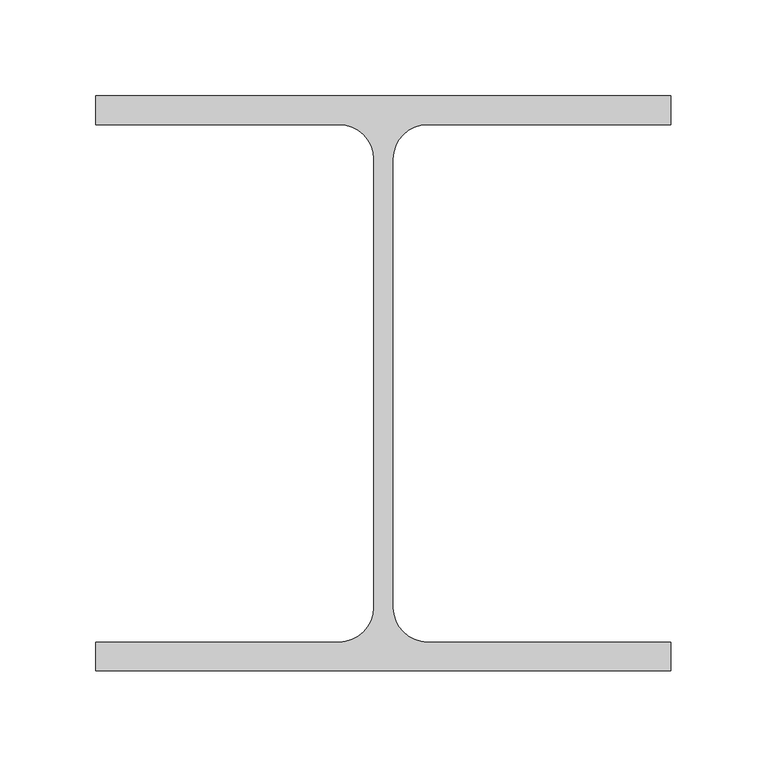
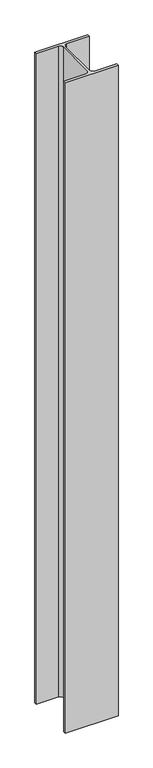
"""IFC4 building model written with IfcOpenShell, lengths in millimetres: column geometry, 0912_Steel Column_H_KSD3502 : H_SC_ASC_H-300x300x10x15."""

from ifc_helpers import new_model, si_unit, point, frame, frame_2d, origin, place, context, project, spatial, polyline, circle_curve, trimmed, segment, composite_curve, outline, extrude, source, transform, mapped, element, save


def column_599e6a97(model_context):
    return source(origin(), model_context, "Body", "SweptSolid", [
        extrude(outline(composite_curve([segment(polyline([(150.0, 150.0), (150.0, 135.0), (23.0, 135.0)]), True, "CONTINUOUS"), segment(trimmed(circle_curve(frame_2d((23.0, 117.0)), 18.0), [point((23.0, 135.0))], [point((5.0, 117.0))], True, "CARTESIAN"), True, "CONTINUOUS"), segment(polyline([(5.0, 117.0), (5.0, -117.0)]), True, "CONTINUOUS"), segment(trimmed(circle_curve(frame_2d((23.0, -117.0)), 18.0), [point((5.0, -117.0))], [point((23.0, -135.0))], True, "CARTESIAN"), True, "CONTINUOUS"), segment(polyline([(23.0, -135.0), (150.0, -135.0), (150.0, -150.0), (-150.0, -150.0), (-150.0, -135.0), (-23.0, -135.0)]), True, "CONTINUOUS"), segment(trimmed(circle_curve(frame_2d((-23.0, -117.0)), 18.0), [point((-23.0, -135.0))], [point((-5.0, -117.0))], True, "CARTESIAN"), True, "CONTINUOUS"), segment(polyline([(-5.0, -117.0), (-5.0, 117.0)]), True, "CONTINUOUS"), segment(trimmed(circle_curve(frame_2d((-23.0, 117.0)), 18.0), [point((-5.0, 117.0))], [point((-23.0, 135.0))], True, "CARTESIAN"), True, "CONTINUOUS"), segment(polyline([(-23.0, 135.0), (-150.0, 135.0), (-150.0, 150.0), (150.0, 150.0)]), True, "CONTINUOUS")], self_intersect=False)), frame((0.0, 0.0, 685.9720055), z_axis=(0.0, 0.0, 1.0), x_axis=(1.0, 0.0, 0.0)), (0.0, 0.0, 1.0), 3914.0),
    ])


if __name__ == "__main__":
    model = new_model("IFC4")
    model_context = context("Model", 3, world=origin())
    ifc_project = project(units=[si_unit("LENGTHUNIT", "METRE", prefix="MILLI")], contexts=[model_context])
    site = spatial("IfcSite", under=ifc_project)
    building = spatial("IfcBuilding", under=site)
    placement = place(None, origin())
    column_shape = column_599e6a97(model_context)
    element("IfcColumn", 1, ObjectType="0912_Steel Column_H_KSD3502 : H_SC_ASC_H-300x300x10x15", at=placement, inside=building, context=model_context, shape_type="MappedRepresentation", body=[
        mapped(column_shape, transform((0.0, 0.0, 0.0), x_axis=(1.0, 0.0, 0.0), y_axis=(0.0, 1.0, 0.0), z_axis=(0.0, 0.0, 1.0))),
    ])
    save(model, "model.ifc")

# Revit data of these elements
# Type "0912_Steel Column_H_KSD3502 : H_SC_ASC_H-300x300x10x15"
#   H_WM Code_1 = "S01AA002-00001 | Main Steel Structure Fabrication Work | Shelter/Building | Medium Steel - Standard (90KG/M>Weight≥30KG/M) | Material: (   )"
#   H_WM Code_2 = "S03AA028-00001 | Main Steel Structure Erection Work | Shelter/Building | Medium Steel (90KG/M>Weight≥30KG/M) | Material: (   )"
#   H_WM Code_3 = "S01AA010-00001 | Main Steel Structure Fabrication Work | Shelter/Building | Steel Painting/Coating | for Non-Fireproofed Steel Surface, Surface Preparation, Primer, Second & Final Coat | Material: (   )"
#   H_Q'ty Cal Type Tag = "SC-Q2"
#   Width = 30.0 cm
#   Web Thickness = 1.0 cm
#   Web Fillet = 1.8 cm
#   Warping Constant = 1370670.0 cm⁶
#   Torsional Moment of Inertia = 77.00 cm⁴
#   Section Area = 119.8 cm²
#   Plastic Modulus weak axis = 684.0 cm³
#   Plastic Modulus strong axis = 1500.0 cm³
#   Perimeter = 1.75 m²/m
#   Nominal Weight = 94.00 kgf/m
#   Moment of Inertia weak axis = 6750.00 cm⁴
#   Moment of Inertia strong axis = 20400.00 cm⁴
#   Height = 30.0 cm
#   Flange Thickness = 1.5 cm
#   Elastic Modulus weak axis = 450.0 cm³
#   Elastic Modulus strong axis = 1360.0 cm³
#   Centroid Vertical = 15.0 cm
#   Centroid Horizontal = 15.0 cm
#   Structural Material [instance default] = Steel, 45-345
#   Section Name Key = ""
#   Bolt Spacing = 0
#   Assembly Code = ""
# Element 1 (IfcColumn, "0912_Steel Column_H_KSD3502 : H_SC_ASC_H-300x300x10x15")
#   Structural Material = none
# Materials
#   "Steel, 45-345": class "Metal", colour RGB 189 187 185, transparency 0, Description = "Steel 345 MPa", Cost = 0
